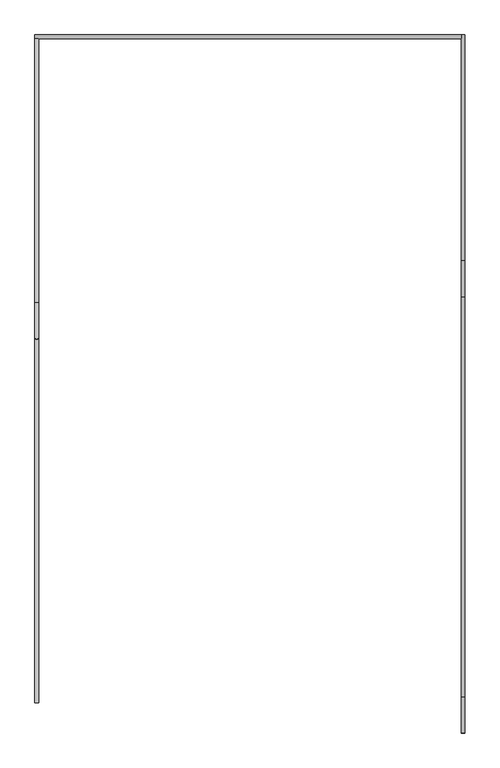
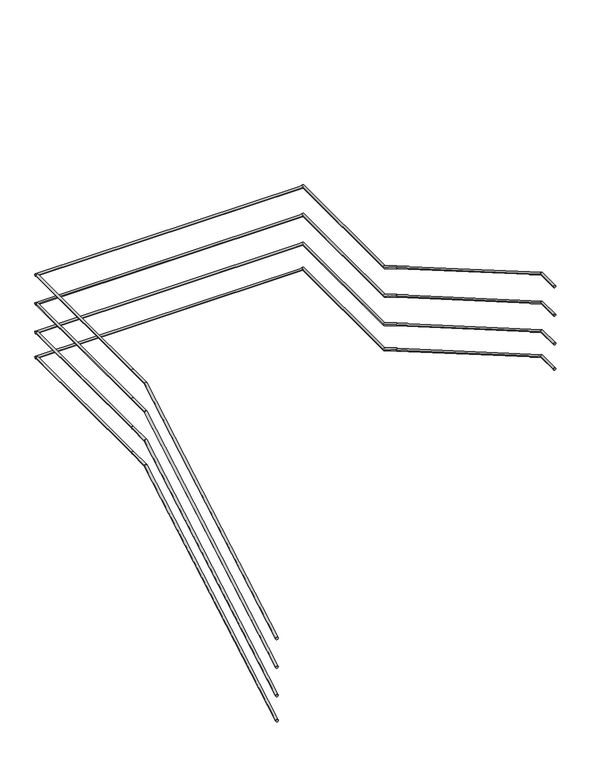
"""IFC4 building model written with IfcOpenShell, lengths in millimetres: railing geometry."""

from ifc_helpers import new_model, si_unit, frame, origin, place, context, project, spatial, circle_curve, ellipse_curve, source, transform, mapped, element, save
from ifc_brep_helpers import plane_surface, cylinder_surface, advanced_brep


def railing_27d6a30b(model_context):
    return source(origin(), model_context, "Body", "AdvancedBrep", [
        advanced_brep(
        [(51115.4, 12029.5208589, 12766.5366726), (51085.4, 12029.5208589, 12766.5366726), (51115.4, 15033.554313, 14508.0053416), (51085.4, 15033.554313, 14508.0053416), (51115.4, 15329.5208589, 14508.0053416), (51085.4, 15329.5208589, 14508.0053416)],
        [
            (0, 1, ellipse_curve(frame((51100.4, 12029.5208589, 12766.5366726), z_axis=(0.0, -1.0, 0.0), x_axis=(0.0, 0.0, -1.0)), 17.3382342, 15.0)),
            (1, 0, ellipse_curve(frame((51100.4, 12029.5208589, 12766.5366726), z_axis=(0.0, -1.0, 0.0), x_axis=(0.0, 0.0, -1.0)), 17.3382342, 15.0)),
            (0, 2),
            (2, 3, ellipse_curve(frame((51100.4, 15033.554313, 14508.0053416), z_axis=(0.0, -0.9656966401166088, -0.25967286971782944), x_axis=(0.0, 0.25967286971782905, -0.9656966401166089)), 15.5328282, 15.0)),
            (3, 1),
            (3, 2, ellipse_curve(frame((51100.4, 15033.554313, 14508.0053416), z_axis=(0.0, -0.9656966401166088, -0.25967286971782944), x_axis=(0.0, 0.25967286971782905, -0.9656966401166089)), 15.5328282, 15.0)),
            (4, 5, circle_curve(frame((51100.4, 15329.5208589, 14508.0053416), z_axis=(0.0, 1.0, 0.0), x_axis=(-1.0, 0.0, 0.0)), 15.0)),
            (5, 4, circle_curve(frame((51100.4, 15329.5208589, 14508.0053416), z_axis=(0.0, 1.0, 0.0), x_axis=(-1.0, 0.0, 0.0)), 15.0)),
            (2, 4),
            (5, 3),
        ],
        [
            plane_surface(frame((51100.4, 12029.5208589, 12783.8749068), z_axis=(0.0, -1.0, 0.0), x_axis=(0.0, 0.0, 1.0))),
            cylinder_surface(frame((51100.4, 12037.0438154, 12770.8978068), z_axis=(0.0, -0.8651400014650144, -0.5015304356318916), x_axis=(-1.0, 0.0, 0.0)), 15.0),
            plane_surface(frame((51100.4, 15329.5208589, 14523.0053416), z_axis=(0.0, 1.0, 0.0), x_axis=(0.0, 0.0, 1.0))),
            cylinder_surface(frame((51100.4, 15029.5208589, 14508.0053416), z_axis=(0.0, -1.0, 0.0), x_axis=(-1.0, 0.0, 0.0)), 15.0),
        ],
        [
            (0, [[1, 2]]),
            (1, [[-1, 3, 4, 5]]),
            (1, [[-2, -5, 6, -3]]),
            (2, [[7, 8]]),
            (3, [[-4, 9, -8, 10]]),
            (3, [[-6, -10, -7, -9]]),
        ],
    ),
        advanced_brep(
        [(51115.4, 15329.5208589, 14508.0053416), (51085.4, 15329.5208589, 14508.0053416), (51115.4, 17509.1208589, 14508.0053416), (51085.4, 17509.1208589, 14508.0053416)],
        [
            (0, 1, circle_curve(frame((51100.4, 15329.5208589, 14508.0053416), z_axis=(0.0, -1.0, 0.0), x_axis=(-1.0, 0.0, 0.0)), 15.0)),
            (1, 0, circle_curve(frame((51100.4, 15329.5208589, 14508.0053416), z_axis=(0.0, -1.0, 0.0), x_axis=(-1.0, 0.0, 0.0)), 15.0)),
            (2, 3, circle_curve(frame((51100.4, 17509.1208589, 14508.0053416), z_axis=(0.0, 1.0, 0.0), x_axis=(-1.0, 0.0, 0.0)), 15.0)),
            (3, 2, circle_curve(frame((51100.4, 17509.1208589, 14508.0053416), z_axis=(0.0, 1.0, 0.0), x_axis=(-1.0, 0.0, 0.0)), 15.0)),
            (0, 2),
            (3, 1),
        ],
        [
            plane_surface(frame((51100.4, 15329.5208589, 14523.0053416), z_axis=(0.0, -1.0, 0.0), x_axis=(0.0, 0.0, 1.0))),
            plane_surface(frame((51100.4, 17509.1208589, 14523.0053416), z_axis=(0.0, 1.0, 0.0), x_axis=(0.0, 0.0, 1.0))),
            cylinder_surface(frame((51100.4, 15329.5208589, 14508.0053416), z_axis=(0.0, -1.0, 0.0), x_axis=(-1.0, 0.0, 0.0)), 15.0),
        ],
        [
            (0, [[1, 2]]),
            (1, [[3, 4]]),
            (2, [[-1, 5, -4, 6]]),
            (2, [[-2, -6, -3, -5]]),
        ],
    ),
        advanced_brep(
        [(51085.4, 17509.1208589, 14508.0053416), (51085.4, 17539.1208589, 14508.0053416), (54606.835546, 17509.1208589, 14508.0053416), (54606.835546, 17539.1208589, 14508.0053416)],
        [
            (0, 1, circle_curve(frame((51085.4, 17524.1208589, 14508.0053416), z_axis=(-1.0, 0.0, 0.0), x_axis=(0.0, 1.0, 0.0)), 15.0)),
            (1, 0, circle_curve(frame((51085.4, 17524.1208589, 14508.0053416), z_axis=(-1.0, 0.0, 0.0), x_axis=(0.0, 1.0, 0.0)), 15.0)),
            (2, 3, circle_curve(frame((54606.835546, 17524.1208589, 14508.0053416), z_axis=(1.0, 0.0, 0.0), x_axis=(0.0, 1.0, 0.0)), 15.0)),
            (3, 2, circle_curve(frame((54606.835546, 17524.1208589, 14508.0053416), z_axis=(1.0, 0.0, 0.0), x_axis=(0.0, 1.0, 0.0)), 15.0)),
            (0, 2),
            (3, 1),
        ],
        [
            plane_surface(frame((51085.4, 17524.1208589, 14523.0053416), z_axis=(-1.0, 0.0, 0.0), x_axis=(0.0, 1.0, 0.0))),
            plane_surface(frame((54606.835546, 17524.1208589, 14523.0053416), z_axis=(1.0, 0.0, 0.0), x_axis=(0.0, 1.0, 0.0))),
            cylinder_surface(frame((51085.4, 17524.1208589, 14508.0053416), z_axis=(-1.0, 0.0, 0.0), x_axis=(0.0, 1.0, 0.0)), 15.0),
        ],
        [
            (0, [[1, 2]]),
            (1, [[3, 4]]),
            (2, [[-1, 5, -4, 6]]),
            (2, [[-2, -6, -3, -5]]),
        ],
    ),
        advanced_brep(
        [(54606.835546, 17539.1208589, 14508.0053416), (54636.835546, 17539.1208589, 14508.0053416), (54606.835546, 15675.4874048, 14508.0053416), (54636.835546, 15675.4874048, 14508.0053416), (54606.835546, 15379.5208589, 14679.5801509), (54636.835546, 15379.5208589, 14679.5801509)],
        [
            (0, 1, circle_curve(frame((54621.835546, 17539.1208589, 14508.0053416), z_axis=(0.0, 1.0, 0.0), x_axis=(1.0, 0.0, 0.0)), 15.0)),
            (1, 0, circle_curve(frame((54621.835546, 17539.1208589, 14508.0053416), z_axis=(0.0, 1.0, 0.0), x_axis=(1.0, 0.0, 0.0)), 15.0)),
            (0, 2),
            (2, 3, ellipse_curve(frame((54621.835546, 15675.4874048, 14508.0053416), z_axis=(0.0, 0.9656966401166088, -0.25967286971782944), x_axis=(0.0, 0.2596728697178298, 0.9656966401166087)), 15.5328282, 15.0)),
            (3, 1),
            (3, 2, ellipse_curve(frame((54621.835546, 15675.4874048, 14508.0053416), z_axis=(0.0, 0.9656966401166088, -0.25967286971782944), x_axis=(0.0, 0.2596728697178298, 0.9656966401166087)), 15.5328282, 15.0)),
            (4, 5, ellipse_curve(frame((54621.835546, 15379.5208589, 14679.5801509), z_axis=(0.0, -1.0, 0.0), x_axis=(0.0, 0.0, -1.0)), 17.3382342, 15.0)),
            (5, 4, ellipse_curve(frame((54621.835546, 15379.5208589, 14679.5801509), z_axis=(0.0, -1.0, 0.0), x_axis=(0.0, 0.0, -1.0)), 17.3382342, 15.0)),
            (2, 4),
            (5, 3),
        ],
        [
            plane_surface(frame((54621.835546, 17539.1208589, 14523.0053416), z_axis=(0.0, 1.0, 0.0), x_axis=(0.0, 0.0, -1.0))),
            cylinder_surface(frame((54621.835546, 17539.1208589, 14508.0053416), z_axis=(0.0, 1.0, 0.0), x_axis=(1.0, 0.0, 0.0)), 15.0),
            plane_surface(frame((54621.835546, 15379.5208589, 14696.9183851), z_axis=(0.0, -1.0, 0.0), x_axis=(0.0, 0.0, -1.0))),
            cylinder_surface(frame((54621.835546, 15671.9979024, 14510.0282416), z_axis=(0.0, 0.8651400014650144, -0.5015304356318916), x_axis=(1.0, 0.0, 0.0)), 15.0),
        ],
        [
            (0, [[1, 2]]),
            (1, [[-1, 3, 4, 5]]),
            (1, [[-2, -5, 6, -3]]),
            (2, [[7, 8]]),
            (3, [[-4, 9, -8, 10]]),
            (3, [[-6, -10, -7, -9]]),
        ],
    ),
        advanced_brep(
        [(54606.835546, 15379.5208589, 14679.5801509), (54636.835546, 15379.5208589, 14679.5801509), (54606.835546, 12075.4874048, 16594.9618634), (54636.835546, 12075.4874048, 16594.9618634), (54606.835546, 11779.5208589, 16594.9618634), (54636.835546, 11779.5208589, 16594.9618634)],
        [
            (0, 1, ellipse_curve(frame((54621.835546, 15379.5208589, 14679.5801509), z_axis=(0.0, 1.0, 0.0), x_axis=(0.0, 0.0, -1.0)), 17.3382342, 15.0)),
            (1, 0, ellipse_curve(frame((54621.835546, 15379.5208589, 14679.5801509), z_axis=(0.0, 1.0, 0.0), x_axis=(0.0, 0.0, -1.0)), 17.3382342, 15.0)),
            (0, 2),
            (2, 3, ellipse_curve(frame((54621.835546, 12075.4874048, 16594.9618634), z_axis=(0.0, 0.9656966401166087, -0.2596728697178297), x_axis=(0.0, -0.259672869717829, -0.9656966401166089)), 15.5328282, 15.0)),
            (3, 1),
            (3, 2, ellipse_curve(frame((54621.835546, 12075.4874048, 16594.9618634), z_axis=(0.0, 0.9656966401166087, -0.2596728697178297), x_axis=(0.0, -0.259672869717829, -0.9656966401166089)), 15.5328282, 15.0)),
            (4, 5, circle_curve(frame((54621.835546, 11779.5208589, 16594.9618634), z_axis=(0.0, -1.0, 0.0), x_axis=(1.0, 0.0, 0.0)), 15.0)),
            (5, 4, circle_curve(frame((54621.835546, 11779.5208589, 16594.9618634), z_axis=(0.0, -1.0, 0.0), x_axis=(1.0, 0.0, 0.0)), 15.0)),
            (2, 4),
            (5, 3),
        ],
        [
            plane_surface(frame((54621.835546, 15379.5208589, 14696.9183851), z_axis=(0.0, 1.0, 0.0), x_axis=(0.0, 0.0, -1.0))),
            cylinder_surface(frame((54621.835546, 15371.9979024, 14683.9412851), z_axis=(0.0, 0.865140001465014, -0.5015304356318923), x_axis=(1.0, 0.0, 0.0)), 15.0),
            plane_surface(frame((54621.835546, 11779.5208589, 16609.9618634), z_axis=(0.0, -1.0, 0.0), x_axis=(0.0, 0.0, -1.0))),
            cylinder_surface(frame((54621.835546, 12079.5208589, 16594.9618634), z_axis=(0.0, 1.0, 0.0), x_axis=(1.0, 0.0, 0.0)), 15.0),
        ],
        [
            (0, [[1, 2]]),
            (1, [[-1, 3, 4, 5]]),
            (1, [[-2, -5, 6, -3]]),
            (2, [[7, 8]]),
            (3, [[-4, 9, -8, 10]]),
            (3, [[-6, -10, -7, -9]]),
        ],
    ),
        advanced_brep(
        [(51115.4, 12029.5208589, 11966.5366726), (51085.4, 12029.5208589, 11966.5366726), (51115.4, 15033.554313, 13708.0053416), (51085.4, 15033.554313, 13708.0053416), (51115.4, 15329.5208589, 13708.0053416), (51085.4, 15329.5208589, 13708.0053416)],
        [
            (0, 1, ellipse_curve(frame((51100.4, 12029.5208589, 11966.5366726), z_axis=(0.0, -1.0, 0.0), x_axis=(0.0, 0.0, -1.0)), 17.3382342, 15.0)),
            (1, 0, ellipse_curve(frame((51100.4, 12029.5208589, 11966.5366726), z_axis=(0.0, -1.0, 0.0), x_axis=(0.0, 0.0, -1.0)), 17.3382342, 15.0)),
            (0, 2),
            (2, 3, ellipse_curve(frame((51100.4, 15033.554313, 13708.0053416), z_axis=(0.0, -0.9656966401166088, -0.25967286971782944), x_axis=(0.0, 0.25967286971782905, -0.9656966401166089)), 15.5328282, 15.0)),
            (3, 1),
            (3, 2, ellipse_curve(frame((51100.4, 15033.554313, 13708.0053416), z_axis=(0.0, -0.9656966401166088, -0.25967286971782944), x_axis=(0.0, 0.25967286971782905, -0.9656966401166089)), 15.5328282, 15.0)),
            (4, 5, circle_curve(frame((51100.4, 15329.5208589, 13708.0053416), z_axis=(0.0, 1.0, 0.0), x_axis=(-1.0, 0.0, 0.0)), 15.0)),
            (5, 4, circle_curve(frame((51100.4, 15329.5208589, 13708.0053416), z_axis=(0.0, 1.0, 0.0), x_axis=(-1.0, 0.0, 0.0)), 15.0)),
            (2, 4),
            (5, 3),
        ],
        [
            plane_surface(frame((51100.4, 12029.5208589, 11983.8749068), z_axis=(0.0, -1.0, 0.0), x_axis=(0.0, 0.0, 1.0))),
            cylinder_surface(frame((51100.4, 12037.0438154, 11970.8978068), z_axis=(0.0, -0.8651400014650144, -0.5015304356318916), x_axis=(-1.0, 0.0, 0.0)), 15.0),
            plane_surface(frame((51100.4, 15329.5208589, 13723.0053416), z_axis=(0.0, 1.0, 0.0), x_axis=(0.0, 0.0, 1.0))),
            cylinder_surface(frame((51100.4, 15029.5208589, 13708.0053416), z_axis=(0.0, -1.0, 0.0), x_axis=(-1.0, 0.0, 0.0)), 15.0),
        ],
        [
            (0, [[1, 2]]),
            (1, [[-1, 3, 4, 5]]),
            (1, [[-2, -5, 6, -3]]),
            (2, [[7, 8]]),
            (3, [[-4, 9, -8, 10]]),
            (3, [[-6, -10, -7, -9]]),
        ],
    ),
        advanced_brep(
        [(51115.4, 15329.5208589, 13708.0053416), (51085.4, 15329.5208589, 13708.0053416), (51115.4, 17509.1208589, 13708.0053416), (51085.4, 17509.1208589, 13708.0053416)],
        [
            (0, 1, circle_curve(frame((51100.4, 15329.5208589, 13708.0053416), z_axis=(0.0, -1.0, 0.0), x_axis=(-1.0, 0.0, 0.0)), 15.0)),
            (1, 0, circle_curve(frame((51100.4, 15329.5208589, 13708.0053416), z_axis=(0.0, -1.0, 0.0), x_axis=(-1.0, 0.0, 0.0)), 15.0)),
            (2, 3, circle_curve(frame((51100.4, 17509.1208589, 13708.0053416), z_axis=(0.0, 1.0, 0.0), x_axis=(-1.0, 0.0, 0.0)), 15.0)),
            (3, 2, circle_curve(frame((51100.4, 17509.1208589, 13708.0053416), z_axis=(0.0, 1.0, 0.0), x_axis=(-1.0, 0.0, 0.0)), 15.0)),
            (0, 2),
            (3, 1),
        ],
        [
            plane_surface(frame((51100.4, 15329.5208589, 13723.0053416), z_axis=(0.0, -1.0, 0.0), x_axis=(0.0, 0.0, 1.0))),
            plane_surface(frame((51100.4, 17509.1208589, 13723.0053416), z_axis=(0.0, 1.0, 0.0), x_axis=(0.0, 0.0, 1.0))),
            cylinder_surface(frame((51100.4, 15329.5208589, 13708.0053416), z_axis=(0.0, -1.0, 0.0), x_axis=(-1.0, 0.0, 0.0)), 15.0),
        ],
        [
            (0, [[1, 2]]),
            (1, [[3, 4]]),
            (2, [[-1, 5, -4, 6]]),
            (2, [[-2, -6, -3, -5]]),
        ],
    ),
        advanced_brep(
        [(51085.4, 17509.1208589, 13708.0053416), (51085.4, 17539.1208589, 13708.0053416), (54606.835546, 17509.1208589, 13708.0053416), (54606.835546, 17539.1208589, 13708.0053416)],
        [
            (0, 1, circle_curve(frame((51085.4, 17524.1208589, 13708.0053416), z_axis=(-1.0, 0.0, 0.0), x_axis=(0.0, 1.0, 0.0)), 15.0)),
            (1, 0, circle_curve(frame((51085.4, 17524.1208589, 13708.0053416), z_axis=(-1.0, 0.0, 0.0), x_axis=(0.0, 1.0, 0.0)), 15.0)),
            (2, 3, circle_curve(frame((54606.835546, 17524.1208589, 13708.0053416), z_axis=(1.0, 0.0, 0.0), x_axis=(0.0, 1.0, 0.0)), 15.0)),
            (3, 2, circle_curve(frame((54606.835546, 17524.1208589, 13708.0053416), z_axis=(1.0, 0.0, 0.0), x_axis=(0.0, 1.0, 0.0)), 15.0)),
            (0, 2),
            (3, 1),
        ],
        [
            plane_surface(frame((51085.4, 17524.1208589, 13723.0053416), z_axis=(-1.0, 0.0, 0.0), x_axis=(0.0, 1.0, 0.0))),
            plane_surface(frame((54606.835546, 17524.1208589, 13723.0053416), z_axis=(1.0, 0.0, 0.0), x_axis=(0.0, 1.0, 0.0))),
            cylinder_surface(frame((51085.4, 17524.1208589, 13708.0053416), z_axis=(-1.0, 0.0, 0.0), x_axis=(0.0, 1.0, 0.0)), 15.0),
        ],
        [
            (0, [[1, 2]]),
            (1, [[3, 4]]),
            (2, [[-1, 5, -4, 6]]),
            (2, [[-2, -6, -3, -5]]),
        ],
    ),
        advanced_brep(
        [(54606.835546, 17539.1208589, 13708.0053416), (54636.835546, 17539.1208589, 13708.0053416), (54606.835546, 15675.4874048, 13708.0053416), (54636.835546, 15675.4874048, 13708.0053416), (54606.835546, 15379.5208589, 13879.5801509), (54636.835546, 15379.5208589, 13879.5801509)],
        [
            (0, 1, circle_curve(frame((54621.835546, 17539.1208589, 13708.0053416), z_axis=(0.0, 1.0, 0.0), x_axis=(1.0, 0.0, 0.0)), 15.0)),
            (1, 0, circle_curve(frame((54621.835546, 17539.1208589, 13708.0053416), z_axis=(0.0, 1.0, 0.0), x_axis=(1.0, 0.0, 0.0)), 15.0)),
            (0, 2),
            (2, 3, ellipse_curve(frame((54621.835546, 15675.4874048, 13708.0053416), z_axis=(0.0, 0.9656966401166088, -0.25967286971782944), x_axis=(0.0, 0.2596728697178298, 0.9656966401166087)), 15.5328282, 15.0)),
            (3, 1),
            (3, 2, ellipse_curve(frame((54621.835546, 15675.4874048, 13708.0053416), z_axis=(0.0, 0.9656966401166088, -0.25967286971782944), x_axis=(0.0, 0.2596728697178298, 0.9656966401166087)), 15.5328282, 15.0)),
            (4, 5, ellipse_curve(frame((54621.835546, 15379.5208589, 13879.5801509), z_axis=(0.0, -1.0, 0.0), x_axis=(0.0, 0.0, -1.0)), 17.3382342, 15.0)),
            (5, 4, ellipse_curve(frame((54621.835546, 15379.5208589, 13879.5801509), z_axis=(0.0, -1.0, 0.0), x_axis=(0.0, 0.0, -1.0)), 17.3382342, 15.0)),
            (2, 4),
            (5, 3),
        ],
        [
            plane_surface(frame((54621.835546, 17539.1208589, 13723.0053416), z_axis=(0.0, 1.0, 0.0), x_axis=(0.0, 0.0, -1.0))),
            cylinder_surface(frame((54621.835546, 17539.1208589, 13708.0053416), z_axis=(0.0, 1.0, 0.0), x_axis=(1.0, 0.0, 0.0)), 15.0),
            plane_surface(frame((54621.835546, 15379.5208589, 13896.9183851), z_axis=(0.0, -1.0, 0.0), x_axis=(0.0, 0.0, -1.0))),
            cylinder_surface(frame((54621.835546, 15671.9979024, 13710.0282416), z_axis=(0.0, 0.8651400014650144, -0.5015304356318916), x_axis=(1.0, 0.0, 0.0)), 15.0),
        ],
        [
            (0, [[1, 2]]),
            (1, [[-1, 3, 4, 5]]),
            (1, [[-2, -5, 6, -3]]),
            (2, [[7, 8]]),
            (3, [[-4, 9, -8, 10]]),
            (3, [[-6, -10, -7, -9]]),
        ],
    ),
        advanced_brep(
        [(54606.835546, 15379.5208589, 13879.5801509), (54636.835546, 15379.5208589, 13879.5801509), (54606.835546, 12075.4874048, 15794.9618634), (54636.835546, 12075.4874048, 15794.9618634), (54606.835546, 11779.5208589, 15794.9618634), (54636.835546, 11779.5208589, 15794.9618634)],
        [
            (0, 1, ellipse_curve(frame((54621.835546, 15379.5208589, 13879.5801509), z_axis=(0.0, 1.0, 0.0), x_axis=(0.0, 0.0, -1.0)), 17.3382342, 15.0)),
            (1, 0, ellipse_curve(frame((54621.835546, 15379.5208589, 13879.5801509), z_axis=(0.0, 1.0, 0.0), x_axis=(0.0, 0.0, -1.0)), 17.3382342, 15.0)),
            (0, 2),
            (2, 3, ellipse_curve(frame((54621.835546, 12075.4874048, 15794.9618634), z_axis=(0.0, 0.9656966401166087, -0.2596728697178297), x_axis=(0.0, -0.259672869717829, -0.9656966401166089)), 15.5328282, 15.0)),
            (3, 1),
            (3, 2, ellipse_curve(frame((54621.835546, 12075.4874048, 15794.9618634), z_axis=(0.0, 0.9656966401166087, -0.2596728697178297), x_axis=(0.0, -0.259672869717829, -0.9656966401166089)), 15.5328282, 15.0)),
            (4, 5, circle_curve(frame((54621.835546, 11779.5208589, 15794.9618634), z_axis=(0.0, -1.0, 0.0), x_axis=(1.0, 0.0, 0.0)), 15.0)),
            (5, 4, circle_curve(frame((54621.835546, 11779.5208589, 15794.9618634), z_axis=(0.0, -1.0, 0.0), x_axis=(1.0, 0.0, 0.0)), 15.0)),
            (2, 4),
            (5, 3),
        ],
        [
            plane_surface(frame((54621.835546, 15379.5208589, 13896.9183851), z_axis=(0.0, 1.0, 0.0), x_axis=(0.0, 0.0, -1.0))),
            cylinder_surface(frame((54621.835546, 15371.9979024, 13883.9412851), z_axis=(0.0, 0.865140001465014, -0.5015304356318923), x_axis=(1.0, 0.0, 0.0)), 15.0),
            plane_surface(frame((54621.835546, 11779.5208589, 15809.9618634), z_axis=(0.0, -1.0, 0.0), x_axis=(0.0, 0.0, -1.0))),
            cylinder_surface(frame((54621.835546, 12079.5208589, 15794.9618634), z_axis=(0.0, 1.0, 0.0), x_axis=(1.0, 0.0, 0.0)), 15.0),
        ],
        [
            (0, [[1, 2]]),
            (1, [[-1, 3, 4, 5]]),
            (1, [[-2, -5, 6, -3]]),
            (2, [[7, 8]]),
            (3, [[-4, 9, -8, 10]]),
            (3, [[-6, -10, -7, -9]]),
        ],
    ),
        advanced_brep(
        [(51115.4, 12029.5208589, 12366.5366726), (51085.4, 12029.5208589, 12366.5366726), (51115.4, 15033.554313, 14108.0053416), (51085.4, 15033.554313, 14108.0053416), (51115.4, 15329.5208589, 14108.0053416), (51085.4, 15329.5208589, 14108.0053416)],
        [
            (0, 1, ellipse_curve(frame((51100.4, 12029.5208589, 12366.5366726), z_axis=(0.0, -1.0, 0.0), x_axis=(0.0, 0.0, -1.0)), 17.3382342, 15.0)),
            (1, 0, ellipse_curve(frame((51100.4, 12029.5208589, 12366.5366726), z_axis=(0.0, -1.0, 0.0), x_axis=(0.0, 0.0, -1.0)), 17.3382342, 15.0)),
            (0, 2),
            (2, 3, ellipse_curve(frame((51100.4, 15033.554313, 14108.0053416), z_axis=(0.0, -0.9656966401166088, -0.25967286971782944), x_axis=(0.0, 0.25967286971782905, -0.9656966401166089)), 15.5328282, 15.0)),
            (3, 1),
            (3, 2, ellipse_curve(frame((51100.4, 15033.554313, 14108.0053416), z_axis=(0.0, -0.9656966401166088, -0.25967286971782944), x_axis=(0.0, 0.25967286971782905, -0.9656966401166089)), 15.5328282, 15.0)),
            (4, 5, circle_curve(frame((51100.4, 15329.5208589, 14108.0053416), z_axis=(0.0, 1.0, 0.0), x_axis=(-1.0, 0.0, 0.0)), 15.0)),
            (5, 4, circle_curve(frame((51100.4, 15329.5208589, 14108.0053416), z_axis=(0.0, 1.0, 0.0), x_axis=(-1.0, 0.0, 0.0)), 15.0)),
            (2, 4),
            (5, 3),
        ],
        [
            plane_surface(frame((51100.4, 12029.5208589, 12383.8749068), z_axis=(0.0, -1.0, 0.0), x_axis=(0.0, 0.0, 1.0))),
            cylinder_surface(frame((51100.4, 12037.0438154, 12370.8978068), z_axis=(0.0, -0.8651400014650144, -0.5015304356318916), x_axis=(-1.0, 0.0, 0.0)), 15.0),
            plane_surface(frame((51100.4, 15329.5208589, 14123.0053416), z_axis=(0.0, 1.0, 0.0), x_axis=(0.0, 0.0, 1.0))),
            cylinder_surface(frame((51100.4, 15029.5208589, 14108.0053416), z_axis=(0.0, -1.0, 0.0), x_axis=(-1.0, 0.0, 0.0)), 15.0),
        ],
        [
            (0, [[1, 2]]),
            (1, [[-1, 3, 4, 5]]),
            (1, [[-2, -5, 6, -3]]),
            (2, [[7, 8]]),
            (3, [[-4, 9, -8, 10]]),
            (3, [[-6, -10, -7, -9]]),
        ],
    ),
        advanced_brep(
        [(51115.4, 15329.5208589, 14108.0053416), (51085.4, 15329.5208589, 14108.0053416), (51115.4, 17509.1208589, 14108.0053416), (51085.4, 17509.1208589, 14108.0053416)],
        [
            (0, 1, circle_curve(frame((51100.4, 15329.5208589, 14108.0053416), z_axis=(0.0, -1.0, 0.0), x_axis=(-1.0, 0.0, 0.0)), 15.0)),
            (1, 0, circle_curve(frame((51100.4, 15329.5208589, 14108.0053416), z_axis=(0.0, -1.0, 0.0), x_axis=(-1.0, 0.0, 0.0)), 15.0)),
            (2, 3, circle_curve(frame((51100.4, 17509.1208589, 14108.0053416), z_axis=(0.0, 1.0, 0.0), x_axis=(-1.0, 0.0, 0.0)), 15.0)),
            (3, 2, circle_curve(frame((51100.4, 17509.1208589, 14108.0053416), z_axis=(0.0, 1.0, 0.0), x_axis=(-1.0, 0.0, 0.0)), 15.0)),
            (0, 2),
            (3, 1),
        ],
        [
            plane_surface(frame((51100.4, 15329.5208589, 14123.0053416), z_axis=(0.0, -1.0, 0.0), x_axis=(0.0, 0.0, 1.0))),
            plane_surface(frame((51100.4, 17509.1208589, 14123.0053416), z_axis=(0.0, 1.0, 0.0), x_axis=(0.0, 0.0, 1.0))),
            cylinder_surface(frame((51100.4, 15329.5208589, 14108.0053416), z_axis=(0.0, -1.0, 0.0), x_axis=(-1.0, 0.0, 0.0)), 15.0),
        ],
        [
            (0, [[1, 2]]),
            (1, [[3, 4]]),
            (2, [[-1, 5, -4, 6]]),
            (2, [[-2, -6, -3, -5]]),
        ],
    ),
        advanced_brep(
        [(51085.4, 17509.1208589, 14108.0053416), (51085.4, 17539.1208589, 14108.0053416), (54606.835546, 17509.1208589, 14108.0053416), (54606.835546, 17539.1208589, 14108.0053416)],
        [
            (0, 1, circle_curve(frame((51085.4, 17524.1208589, 14108.0053416), z_axis=(-1.0, 0.0, 0.0), x_axis=(0.0, 1.0, 0.0)), 15.0)),
            (1, 0, circle_curve(frame((51085.4, 17524.1208589, 14108.0053416), z_axis=(-1.0, 0.0, 0.0), x_axis=(0.0, 1.0, 0.0)), 15.0)),
            (2, 3, circle_curve(frame((54606.835546, 17524.1208589, 14108.0053416), z_axis=(1.0, 0.0, 0.0), x_axis=(0.0, 1.0, 0.0)), 15.0)),
            (3, 2, circle_curve(frame((54606.835546, 17524.1208589, 14108.0053416), z_axis=(1.0, 0.0, 0.0), x_axis=(0.0, 1.0, 0.0)), 15.0)),
            (0, 2),
            (3, 1),
        ],
        [
            plane_surface(frame((51085.4, 17524.1208589, 14123.0053416), z_axis=(-1.0, 0.0, 0.0), x_axis=(0.0, 1.0, 0.0))),
            plane_surface(frame((54606.835546, 17524.1208589, 14123.0053416), z_axis=(1.0, 0.0, 0.0), x_axis=(0.0, 1.0, 0.0))),
            cylinder_surface(frame((51085.4, 17524.1208589, 14108.0053416), z_axis=(-1.0, 0.0, 0.0), x_axis=(0.0, 1.0, 0.0)), 15.0),
        ],
        [
            (0, [[1, 2]]),
            (1, [[3, 4]]),
            (2, [[-1, 5, -4, 6]]),
            (2, [[-2, -6, -3, -5]]),
        ],
    ),
        advanced_brep(
        [(54606.835546, 17539.1208589, 14108.0053416), (54636.835546, 17539.1208589, 14108.0053416), (54606.835546, 15675.4874048, 14108.0053416), (54636.835546, 15675.4874048, 14108.0053416), (54606.835546, 15379.5208589, 14279.5801509), (54636.835546, 15379.5208589, 14279.5801509)],
        [
            (0, 1, circle_curve(frame((54621.835546, 17539.1208589, 14108.0053416), z_axis=(0.0, 1.0, 0.0), x_axis=(1.0, 0.0, 0.0)), 15.0)),
            (1, 0, circle_curve(frame((54621.835546, 17539.1208589, 14108.0053416), z_axis=(0.0, 1.0, 0.0), x_axis=(1.0, 0.0, 0.0)), 15.0)),
            (0, 2),
            (2, 3, ellipse_curve(frame((54621.835546, 15675.4874048, 14108.0053416), z_axis=(0.0, 0.9656966401166088, -0.25967286971782944), x_axis=(0.0, 0.2596728697178298, 0.9656966401166087)), 15.5328282, 15.0)),
            (3, 1),
            (3, 2, ellipse_curve(frame((54621.835546, 15675.4874048, 14108.0053416), z_axis=(0.0, 0.9656966401166088, -0.25967286971782944), x_axis=(0.0, 0.2596728697178298, 0.9656966401166087)), 15.5328282, 15.0)),
            (4, 5, ellipse_curve(frame((54621.835546, 15379.5208589, 14279.5801509), z_axis=(0.0, -1.0, 0.0), x_axis=(0.0, 0.0, -1.0)), 17.3382342, 15.0)),
            (5, 4, ellipse_curve(frame((54621.835546, 15379.5208589, 14279.5801509), z_axis=(0.0, -1.0, 0.0), x_axis=(0.0, 0.0, -1.0)), 17.3382342, 15.0)),
            (2, 4),
            (5, 3),
        ],
        [
            plane_surface(frame((54621.835546, 17539.1208589, 14123.0053416), z_axis=(0.0, 1.0, 0.0), x_axis=(0.0, 0.0, -1.0))),
            cylinder_surface(frame((54621.835546, 17539.1208589, 14108.0053416), z_axis=(0.0, 1.0, 0.0), x_axis=(1.0, 0.0, 0.0)), 15.0),
            plane_surface(frame((54621.835546, 15379.5208589, 14296.9183851), z_axis=(0.0, -1.0, 0.0), x_axis=(0.0, 0.0, -1.0))),
            cylinder_surface(frame((54621.835546, 15671.9979024, 14110.0282416), z_axis=(0.0, 0.8651400014650144, -0.5015304356318916), x_axis=(1.0, 0.0, 0.0)), 15.0),
        ],
        [
            (0, [[1, 2]]),
            (1, [[-1, 3, 4, 5]]),
            (1, [[-2, -5, 6, -3]]),
            (2, [[7, 8]]),
            (3, [[-4, 9, -8, 10]]),
            (3, [[-6, -10, -7, -9]]),
        ],
    ),
        advanced_brep(
        [(54606.835546, 15379.5208589, 14279.5801509), (54636.835546, 15379.5208589, 14279.5801509), (54606.835546, 12075.4874048, 16194.9618634), (54636.835546, 12075.4874048, 16194.9618634), (54606.835546, 11779.5208589, 16194.9618634), (54636.835546, 11779.5208589, 16194.9618634)],
        [
            (0, 1, ellipse_curve(frame((54621.835546, 15379.5208589, 14279.5801509), z_axis=(0.0, 1.0, 0.0), x_axis=(0.0, 0.0, -1.0)), 17.3382342, 15.0)),
            (1, 0, ellipse_curve(frame((54621.835546, 15379.5208589, 14279.5801509), z_axis=(0.0, 1.0, 0.0), x_axis=(0.0, 0.0, -1.0)), 17.3382342, 15.0)),
            (0, 2),
            (2, 3, ellipse_curve(frame((54621.835546, 12075.4874048, 16194.9618634), z_axis=(0.0, 0.9656966401166087, -0.2596728697178297), x_axis=(0.0, -0.259672869717829, -0.9656966401166089)), 15.5328282, 15.0)),
            (3, 1),
            (3, 2, ellipse_curve(frame((54621.835546, 12075.4874048, 16194.9618634), z_axis=(0.0, 0.9656966401166087, -0.2596728697178297), x_axis=(0.0, -0.259672869717829, -0.9656966401166089)), 15.5328282, 15.0)),
            (4, 5, circle_curve(frame((54621.835546, 11779.5208589, 16194.9618634), z_axis=(0.0, -1.0, 0.0), x_axis=(1.0, 0.0, 0.0)), 15.0)),
            (5, 4, circle_curve(frame((54621.835546, 11779.5208589, 16194.9618634), z_axis=(0.0, -1.0, 0.0), x_axis=(1.0, 0.0, 0.0)), 15.0)),
            (2, 4),
            (5, 3),
        ],
        [
            plane_surface(frame((54621.835546, 15379.5208589, 14296.9183851), z_axis=(0.0, 1.0, 0.0), x_axis=(0.0, 0.0, -1.0))),
            cylinder_surface(frame((54621.835546, 15371.9979024, 14283.9412851), z_axis=(0.0, 0.865140001465014, -0.5015304356318923), x_axis=(1.0, 0.0, 0.0)), 15.0),
            plane_surface(frame((54621.835546, 11779.5208589, 16209.9618634), z_axis=(0.0, -1.0, 0.0), x_axis=(0.0, 0.0, -1.0))),
            cylinder_surface(frame((54621.835546, 12079.5208589, 16194.9618634), z_axis=(0.0, 1.0, 0.0), x_axis=(1.0, 0.0, 0.0)), 15.0),
        ],
        [
            (0, [[1, 2]]),
            (1, [[-1, 3, 4, 5]]),
            (1, [[-2, -5, 6, -3]]),
            (2, [[7, 8]]),
            (3, [[-4, 9, -8, 10]]),
            (3, [[-6, -10, -7, -9]]),
        ],
    ),
        advanced_brep(
        [(51115.4, 12029.5208589, 11616.5366726), (51085.4, 12029.5208589, 11616.5366726), (51115.4, 15033.554313, 13358.0053416), (51085.4, 15033.554313, 13358.0053416), (51115.4, 15329.5208589, 13358.0053416), (51085.4, 15329.5208589, 13358.0053416)],
        [
            (0, 1, ellipse_curve(frame((51100.4, 12029.5208589, 11616.5366726), z_axis=(0.0, -1.0, 0.0), x_axis=(0.0, 0.0, -1.0)), 17.3382342, 15.0)),
            (1, 0, ellipse_curve(frame((51100.4, 12029.5208589, 11616.5366726), z_axis=(0.0, -1.0, 0.0), x_axis=(0.0, 0.0, -1.0)), 17.3382342, 15.0)),
            (0, 2),
            (2, 3, ellipse_curve(frame((51100.4, 15033.554313, 13358.0053416), z_axis=(0.0, -0.9656966401166088, -0.25967286971782944), x_axis=(0.0, 0.25967286971782905, -0.9656966401166089)), 15.5328282, 15.0)),
            (3, 1),
            (3, 2, ellipse_curve(frame((51100.4, 15033.554313, 13358.0053416), z_axis=(0.0, -0.9656966401166088, -0.25967286971782944), x_axis=(0.0, 0.25967286971782905, -0.9656966401166089)), 15.5328282, 15.0)),
            (4, 5, circle_curve(frame((51100.4, 15329.5208589, 13358.0053416), z_axis=(0.0, 1.0, 0.0), x_axis=(-1.0, 0.0, 0.0)), 15.0)),
            (5, 4, circle_curve(frame((51100.4, 15329.5208589, 13358.0053416), z_axis=(0.0, 1.0, 0.0), x_axis=(-1.0, 0.0, 0.0)), 15.0)),
            (2, 4),
            (5, 3),
        ],
        [
            plane_surface(frame((51100.4, 12029.5208589, 11633.8749068), z_axis=(0.0, -1.0, 0.0), x_axis=(0.0, 0.0, 1.0))),
            cylinder_surface(frame((51100.4, 12037.0438154, 11620.8978068), z_axis=(0.0, -0.8651400014650144, -0.5015304356318916), x_axis=(-1.0, 0.0, 0.0)), 15.0),
            plane_surface(frame((51100.4, 15329.5208589, 13373.0053416), z_axis=(0.0, 1.0, 0.0), x_axis=(0.0, 0.0, 1.0))),
            cylinder_surface(frame((51100.4, 15029.5208589, 13358.0053416), z_axis=(0.0, -1.0, 0.0), x_axis=(-1.0, 0.0, 0.0)), 15.0),
        ],
        [
            (0, [[1, 2]]),
            (1, [[-1, 3, 4, 5]]),
            (1, [[-2, -5, 6, -3]]),
            (2, [[7, 8]]),
            (3, [[-4, 9, -8, 10]]),
            (3, [[-6, -10, -7, -9]]),
        ],
    ),
        advanced_brep(
        [(51115.4, 15329.5208589, 13358.0053416), (51085.4, 15329.5208589, 13358.0053416), (51115.4, 17509.1208589, 13358.0053416), (51085.4, 17509.1208589, 13358.0053416)],
        [
            (0, 1, circle_curve(frame((51100.4, 15329.5208589, 13358.0053416), z_axis=(0.0, -1.0, 0.0), x_axis=(-1.0, 0.0, 0.0)), 15.0)),
            (1, 0, circle_curve(frame((51100.4, 15329.5208589, 13358.0053416), z_axis=(0.0, -1.0, 0.0), x_axis=(-1.0, 0.0, 0.0)), 15.0)),
            (2, 3, circle_curve(frame((51100.4, 17509.1208589, 13358.0053416), z_axis=(0.0, 1.0, 0.0), x_axis=(-1.0, 0.0, 0.0)), 15.0)),
            (3, 2, circle_curve(frame((51100.4, 17509.1208589, 13358.0053416), z_axis=(0.0, 1.0, 0.0), x_axis=(-1.0, 0.0, 0.0)), 15.0)),
            (0, 2),
            (3, 1),
        ],
        [
            plane_surface(frame((51100.4, 15329.5208589, 13373.0053416), z_axis=(0.0, -1.0, 0.0), x_axis=(0.0, 0.0, 1.0))),
            plane_surface(frame((51100.4, 17509.1208589, 13373.0053416), z_axis=(0.0, 1.0, 0.0), x_axis=(0.0, 0.0, 1.0))),
            cylinder_surface(frame((51100.4, 15329.5208589, 13358.0053416), z_axis=(0.0, -1.0, 0.0), x_axis=(-1.0, 0.0, 0.0)), 15.0),
        ],
        [
            (0, [[1, 2]]),
            (1, [[3, 4]]),
            (2, [[-1, 5, -4, 6]]),
            (2, [[-2, -6, -3, -5]]),
        ],
    ),
        advanced_brep(
        [(51085.4, 17509.1208589, 13358.0053416), (51085.4, 17539.1208589, 13358.0053416), (54606.835546, 17509.1208589, 13358.0053416), (54606.835546, 17539.1208589, 13358.0053416)],
        [
            (0, 1, circle_curve(frame((51085.4, 17524.1208589, 13358.0053416), z_axis=(-1.0, 0.0, 0.0), x_axis=(0.0, 1.0, 0.0)), 15.0)),
            (1, 0, circle_curve(frame((51085.4, 17524.1208589, 13358.0053416), z_axis=(-1.0, 0.0, 0.0), x_axis=(0.0, 1.0, 0.0)), 15.0)),
            (2, 3, circle_curve(frame((54606.835546, 17524.1208589, 13358.0053416), z_axis=(1.0, 0.0, 0.0), x_axis=(0.0, 1.0, 0.0)), 15.0)),
            (3, 2, circle_curve(frame((54606.835546, 17524.1208589, 13358.0053416), z_axis=(1.0, 0.0, 0.0), x_axis=(0.0, 1.0, 0.0)), 15.0)),
            (0, 2),
            (3, 1),
        ],
        [
            plane_surface(frame((51085.4, 17524.1208589, 13373.0053416), z_axis=(-1.0, 0.0, 0.0), x_axis=(0.0, 1.0, 0.0))),
            plane_surface(frame((54606.835546, 17524.1208589, 13373.0053416), z_axis=(1.0, 0.0, 0.0), x_axis=(0.0, 1.0, 0.0))),
            cylinder_surface(frame((51085.4, 17524.1208589, 13358.0053416), z_axis=(-1.0, 0.0, 0.0), x_axis=(0.0, 1.0, 0.0)), 15.0),
        ],
        [
            (0, [[1, 2]]),
            (1, [[3, 4]]),
            (2, [[-1, 5, -4, 6]]),
            (2, [[-2, -6, -3, -5]]),
        ],
    ),
        advanced_brep(
        [(54606.835546, 17539.1208589, 13358.0053416), (54636.835546, 17539.1208589, 13358.0053416), (54606.835546, 15675.4874048, 13358.0053416), (54636.835546, 15675.4874048, 13358.0053416), (54606.835546, 15379.5208589, 13529.5801509), (54636.835546, 15379.5208589, 13529.5801509)],
        [
            (0, 1, circle_curve(frame((54621.835546, 17539.1208589, 13358.0053416), z_axis=(0.0, 1.0, 0.0), x_axis=(1.0, 0.0, 0.0)), 15.0)),
            (1, 0, circle_curve(frame((54621.835546, 17539.1208589, 13358.0053416), z_axis=(0.0, 1.0, 0.0), x_axis=(1.0, 0.0, 0.0)), 15.0)),
            (0, 2),
            (2, 3, ellipse_curve(frame((54621.835546, 15675.4874048, 13358.0053416), z_axis=(0.0, 0.9656966401166088, -0.25967286971782944), x_axis=(0.0, 0.2596728697178298, 0.9656966401166087)), 15.5328282, 15.0)),
            (3, 1),
            (3, 2, ellipse_curve(frame((54621.835546, 15675.4874048, 13358.0053416), z_axis=(0.0, 0.9656966401166088, -0.25967286971782944), x_axis=(0.0, 0.2596728697178298, 0.9656966401166087)), 15.5328282, 15.0)),
            (4, 5, ellipse_curve(frame((54621.835546, 15379.5208589, 13529.5801509), z_axis=(0.0, -1.0, 0.0), x_axis=(0.0, 0.0, -1.0)), 17.3382342, 15.0)),
            (5, 4, ellipse_curve(frame((54621.835546, 15379.5208589, 13529.5801509), z_axis=(0.0, -1.0, 0.0), x_axis=(0.0, 0.0, -1.0)), 17.3382342, 15.0)),
            (2, 4),
            (5, 3),
        ],
        [
            plane_surface(frame((54621.835546, 17539.1208589, 13373.0053416), z_axis=(0.0, 1.0, 0.0), x_axis=(0.0, 0.0, -1.0))),
            cylinder_surface(frame((54621.835546, 17539.1208589, 13358.0053416), z_axis=(0.0, 1.0, 0.0), x_axis=(1.0, 0.0, 0.0)), 15.0),
            plane_surface(frame((54621.835546, 15379.5208589, 13546.9183851), z_axis=(0.0, -1.0, 0.0), x_axis=(0.0, 0.0, -1.0))),
            cylinder_surface(frame((54621.835546, 15671.9979024, 13360.0282416), z_axis=(0.0, 0.8651400014650144, -0.5015304356318916), x_axis=(1.0, 0.0, 0.0)), 15.0),
        ],
        [
            (0, [[1, 2]]),
            (1, [[-1, 3, 4, 5]]),
            (1, [[-2, -5, 6, -3]]),
            (2, [[7, 8]]),
            (3, [[-4, 9, -8, 10]]),
            (3, [[-6, -10, -7, -9]]),
        ],
    ),
        advanced_brep(
        [(54606.835546, 15379.5208589, 13529.5801509), (54636.835546, 15379.5208589, 13529.5801509), (54606.835546, 12075.4874048, 15444.9618634), (54636.835546, 12075.4874048, 15444.9618634), (54606.835546, 11779.5208589, 15444.9618634), (54636.835546, 11779.5208589, 15444.9618634)],
        [
            (0, 1, ellipse_curve(frame((54621.835546, 15379.5208589, 13529.5801509), z_axis=(0.0, 1.0, 0.0), x_axis=(0.0, 0.0, -1.0)), 17.3382342, 15.0)),
            (1, 0, ellipse_curve(frame((54621.835546, 15379.5208589, 13529.5801509), z_axis=(0.0, 1.0, 0.0), x_axis=(0.0, 0.0, -1.0)), 17.3382342, 15.0)),
            (0, 2),
            (2, 3, ellipse_curve(frame((54621.835546, 12075.4874048, 15444.9618634), z_axis=(0.0, 0.9656966401166087, -0.2596728697178297), x_axis=(0.0, -0.259672869717829, -0.9656966401166089)), 15.5328282, 15.0)),
            (3, 1),
            (3, 2, ellipse_curve(frame((54621.835546, 12075.4874048, 15444.9618634), z_axis=(0.0, 0.9656966401166087, -0.2596728697178297), x_axis=(0.0, -0.259672869717829, -0.9656966401166089)), 15.5328282, 15.0)),
            (4, 5, circle_curve(frame((54621.835546, 11779.5208589, 15444.9618634), z_axis=(0.0, -1.0, 0.0), x_axis=(1.0, 0.0, 0.0)), 15.0)),
            (5, 4, circle_curve(frame((54621.835546, 11779.5208589, 15444.9618634), z_axis=(0.0, -1.0, 0.0), x_axis=(1.0, 0.0, 0.0)), 15.0)),
            (2, 4),
            (5, 3),
        ],
        [
            plane_surface(frame((54621.835546, 15379.5208589, 13546.9183851), z_axis=(0.0, 1.0, 0.0), x_axis=(0.0, 0.0, -1.0))),
            cylinder_surface(frame((54621.835546, 15371.9979024, 13533.9412851), z_axis=(0.0, 0.865140001465014, -0.5015304356318923), x_axis=(1.0, 0.0, 0.0)), 15.0),
            plane_surface(frame((54621.835546, 11779.5208589, 15459.9618634), z_axis=(0.0, -1.0, 0.0), x_axis=(0.0, 0.0, -1.0))),
            cylinder_surface(frame((54621.835546, 12079.5208589, 15444.9618634), z_axis=(0.0, 1.0, 0.0), x_axis=(1.0, 0.0, 0.0)), 15.0),
        ],
        [
            (0, [[1, 2]]),
            (1, [[-1, 3, 4, 5]]),
            (1, [[-2, -5, 6, -3]]),
            (2, [[7, 8]]),
            (3, [[-4, 9, -8, 10]]),
            (3, [[-6, -10, -7, -9]]),
        ],
    ),
    ])


if __name__ == "__main__":
    model = new_model("IFC4")
    model_context = context("Model", 3, world=origin())
    ifc_project = project(units=[si_unit("LENGTHUNIT", "METRE", prefix="MILLI")], contexts=[model_context])
    site = spatial("IfcSite", under=ifc_project)
    building = spatial("IfcBuilding", under=site)
    placement = place(None, origin())
    railing_shape = railing_27d6a30b(model_context)
    element("IfcRailing", 1, at=placement, inside=building, context=model_context, shape_type="MappedRepresentation", body=[
        mapped(railing_shape, transform((0.0, 0.0, 0.0), x_axis=(1.0, 0.0, 0.0), y_axis=(0.0, 1.0, 0.0), z_axis=(0.0, 0.0, 1.0))),
    ])
    save(model, "model.ifc")
